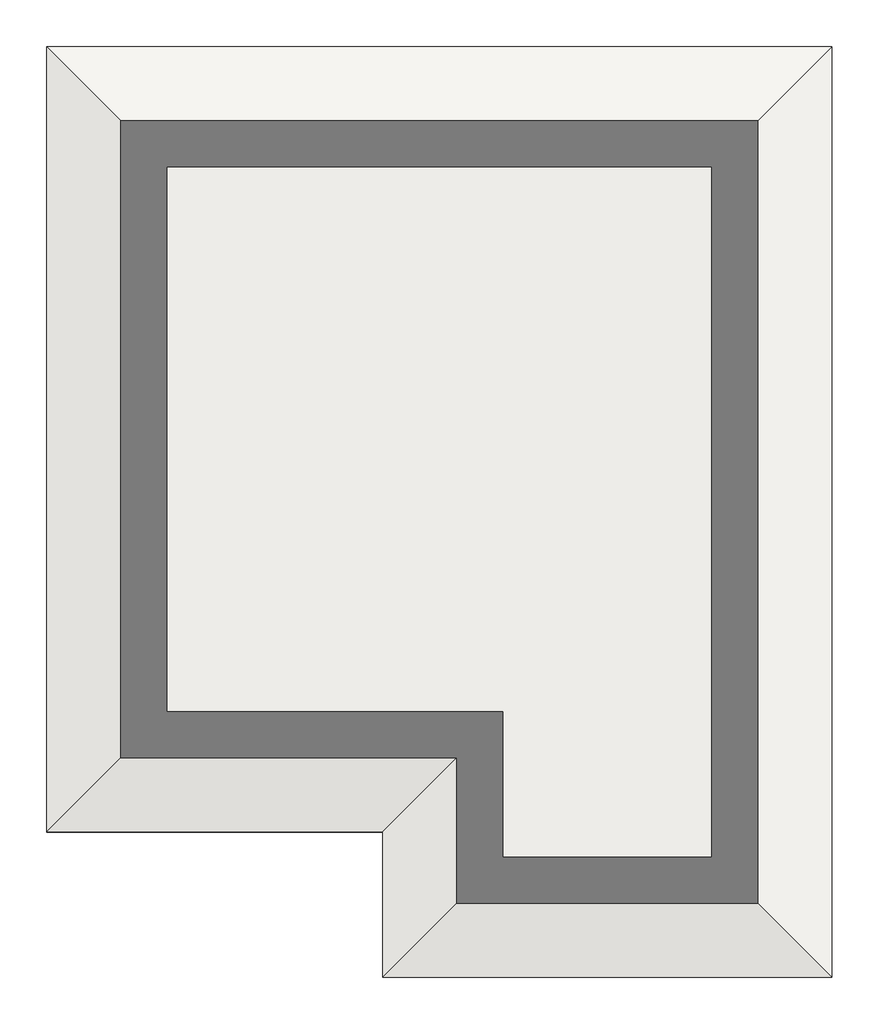
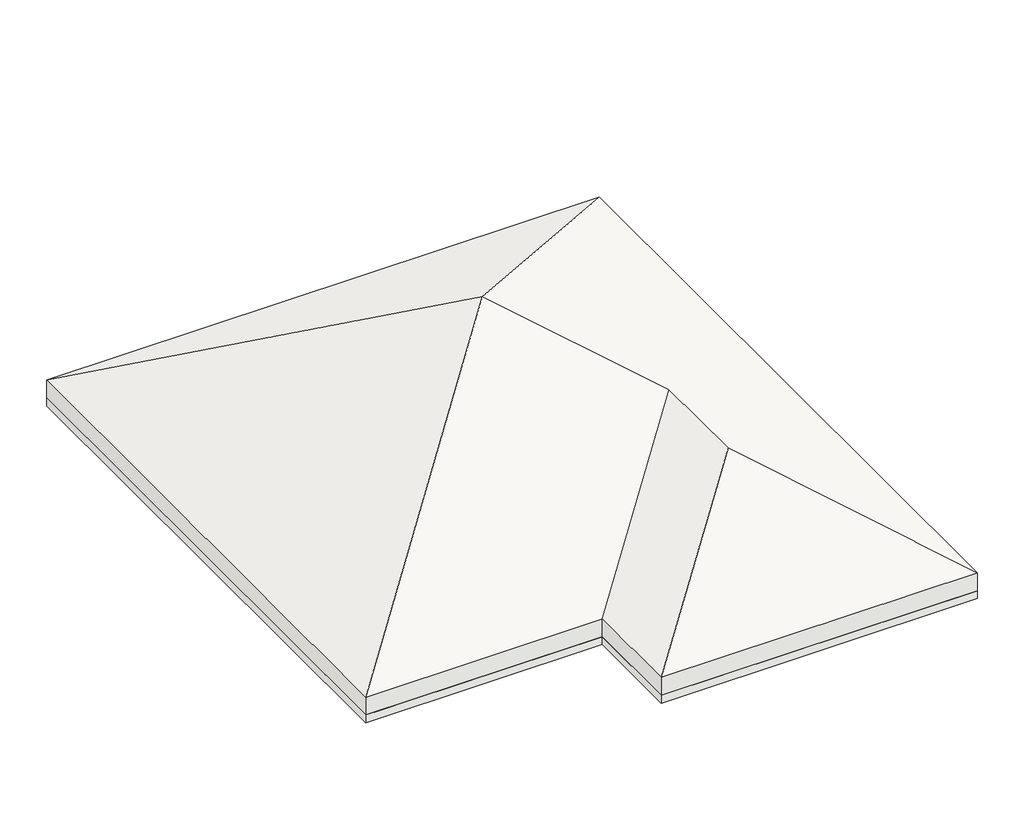
# One storey: 15 beams, 6 walls, 1 roof, 1 slab.
"""IFC4 building model written with IfcOpenShell, lengths in millimetres."""

from ifc_helpers import new_model, si_unit, frame, origin, place, context, project, spatial, polyline, outline, extrude, faceted_brep, element, save

model = new_model("IFC4")

# Units and contexts
model_context = context("Model", 3, world=origin())
ifc_project = project(units=[si_unit("LENGTHUNIT", "METRE", prefix="MILLI")], contexts=[model_context])

# Site, building, storey
site = spatial("IfcSite", under=ifc_project)
building = spatial("IfcBuilding", under=site)
storey = spatial("IfcBuildingStorey", under=building, Name="02 Çatı Katı", Elevation=100780.0)

# Beams
placement = place(None, origin())
element("IfcBeam", 1, ObjectType="M_Concrete-Rectangular Beam : 45x60cm Kiriş", at=placement, inside=storey, context=model_context, shape_type="SweptSolid", body=[
    extrude(outline(polyline([(450.0, 15000.0), (6225.0, 15000.0), (6225.0, 14999.2150597), (5700.0, 14999.2150597), (5700.0, 14550.0), (450.0, 14550.0), (450.0, 15000.0)])), frame((0.0, 0.0, 100180.0), z_axis=(0.0, 0.0, 1.0), x_axis=(1.0, 0.0, 0.0)), (0.0, 0.0, 1.0), 400.0),
])
element("IfcBeam", 2, ObjectType="M_Concrete-Rectangular Beam : 45x60cm Kiriş", at=placement, inside=storey, context=model_context, shape_type="SweptSolid", body=[
    extrude(outline(polyline([(450.0, 8750.0), (5775.0, 8750.0), (5775.0, 8300.0), (450.0, 8300.0), (450.0, 8750.0)])), frame((0.0, 0.0, 100180.0), z_axis=(0.0, 0.0, 1.0), x_axis=(1.0, 0.0, 0.0)), (0.0, 0.0, 1.0), 400.0),
])
element("IfcBeam", 3, ObjectType="M_Concrete-Rectangular Beam : 45x60cm Kiriş", at=placement, inside=storey, context=model_context, shape_type="SweptSolid", body=[
    extrude(outline(polyline([(0.0, 8800.0), (0.0, 14400.0), (450.0, 14400.0), (450.0, 8800.0), (0.0, 8800.0)])), frame((0.0, 0.0, 100180.0), z_axis=(0.0, 0.0, 1.0), x_axis=(1.0, 0.0, 0.0)), (0.0, 0.0, 1.0), 400.0),
])
element("IfcBeam", 4, ObjectType="M_Concrete-Rectangular Beam : 45x60cm Kiriş", at=placement, inside=storey, context=model_context, shape_type="SweptSolid", body=[
    extrude(outline(polyline([(0.0, 3100.0), (0.0, 8200.0), (450.0, 8200.0), (450.0, 3100.0), (0.0, 3100.0)])), frame((0.0, 0.0, 100180.0), z_axis=(0.0, 0.0, 1.0), x_axis=(1.0, 0.0, 0.0)), (0.0, 0.0, 1.0), 400.0),
])
element("IfcBeam", 5, ObjectType="M_Concrete-Rectangular Beam : 45x60cm Kiriş", at=placement, inside=storey, context=model_context, shape_type="SweptSolid", body=[
    extrude(outline(polyline([(5700.0, 2500.0), (450.0, 2500.0), (450.0, 2950.0), (5700.0, 2950.0), (5700.0, 2500.0)])), frame((0.0, 0.0, 100180.0), z_axis=(0.0, 0.0, 1.0), x_axis=(1.0, 0.0, 0.0)), (0.0, 0.0, 1.0), 400.0),
])
element("IfcBeam", 6, ObjectType="M_Concrete-Rectangular Beam : 45x60cm Kiriş", at=placement, inside=storey, context=model_context, shape_type="SweptSolid", body=[
    extrude(outline(polyline([(12050.0, 2500.0), (6300.0, 2500.0), (6300.0, 2950.0), (12050.0, 2950.0), (12050.0, 2500.0)])), frame((0.0, 0.0, 100180.0), z_axis=(0.0, 0.0, 1.0), x_axis=(1.0, 0.0, 0.0)), (0.0, 0.0, 1.0), 400.0),
])
element("IfcBeam", 7, ObjectType="M_Concrete-Rectangular Beam : 45x60cm Kiriş", at=placement, inside=storey, context=model_context, shape_type="SweptSolid", body=[
    extrude(outline(polyline([(12500.0, 8750.0), (12500.0, 3100.0), (12050.0, 3100.0), (12050.0, 8200.0), (12494.8117928, 8200.0), (12494.8117928, 8750.0), (12500.0, 8750.0)])), frame((0.0, 0.0, 100180.0), z_axis=(0.0, 0.0, 1.0), x_axis=(1.0, 0.0, 0.0)), (0.0, 0.0, 1.0), 400.0),
])
element("IfcBeam", 8, ObjectType="M_Concrete-Rectangular Beam : 45x60cm Kiriş", at=placement, inside=storey, context=model_context, shape_type="SweptSolid", body=[
    extrude(outline(polyline([(12032.1117928, 8750.0), (12032.1117928, 8300.0), (6237.7, 8300.0), (6237.7, 8750.0), (12032.1117928, 8750.0)])), frame((0.0, 0.0, 100180.0), z_axis=(0.0, 0.0, 1.0), x_axis=(1.0, 0.0, 0.0)), (0.0, 0.0, 1.0), 400.0),
])
element("IfcBeam", 9, ObjectType="M_Concrete-Rectangular Beam : 30x60cm Kiriş", at=placement, inside=storey, context=model_context, shape_type="SweptSolid", body=[
    extrude(outline(polyline([(9850.0, 15000.0), (9850.0, 14700.0), (6300.0, 14700.0), (6300.0, 15000.0), (9850.0, 15000.0)])), frame((0.0, 0.0, 100180.0), z_axis=(0.0, 0.0, 1.0), x_axis=(1.0, 0.0, 0.0)), (0.0, 0.0, 1.0), 400.0),
])
element("IfcBeam", 10, ObjectType="M_Concrete-Rectangular Beam : 30x60cm Kiriş", at=placement, inside=storey, context=model_context, shape_type="SweptSolid", body=[
    extrude(outline(polyline([(12200.0, 10850.0), (12500.0, 10850.0), (12500.0, 8800.0), (12200.0, 8800.0), (12200.0, 10850.0)])), frame((0.0, 0.0, 100180.0), z_axis=(0.0, 0.0, 1.0), x_axis=(1.0, 0.0, 0.0)), (0.0, 0.0, 1.0), 400.0),
])
element("IfcBeam", 11, ObjectType="M_Concrete-Rectangular Beam : 45x60cm Kiriş", at=placement, inside=storey, context=model_context, shape_type="SweptSolid", body=[
    extrude(outline(polyline([(5775.0, 2950.0), (5775.0, 8200.0), (6225.0, 8200.0), (6225.0, 2950.0), (5775.0, 2950.0)])), frame((0.0, 0.0, 100180.0), z_axis=(0.0, 0.0, 1.0), x_axis=(1.0, 0.0, 0.0)), (0.0, 0.0, 1.0), 400.0),
])
element("IfcBeam", 12, ObjectType="M_Concrete-Rectangular Beam : 45x60cm Kiriş", at=placement, inside=storey, context=model_context, shape_type="SweptSolid", body=[
    extrude(outline(polyline([(5775.0, 14536.5150597), (6225.0, 14536.5150597), (6225.0, 8800.0), (5775.0, 8800.0), (5775.0, 14536.5150597)])), frame((0.0, 0.0, 100180.0), z_axis=(0.0, 0.0, 1.0), x_axis=(1.0, 0.0, 0.0)), (0.0, 0.0, 1.0), 400.0),
])
element("IfcBeam", 13, ObjectType="M_Concrete-Rectangular Beam : 45x60cm Kiriş", at=placement, inside=storey, context=model_context, shape_type="Brep", body=[
    faceted_brep([(5775.0, 2500.0, 100180.0), (5775.0, 400.0, 100180.0), (5775.0, 400.0, 100580.0), (5775.0, 2500.0, 100580.0), (6225.0, 2500.0, 100180.0), (6225.0, 450.0, 100180.0), (6225.0, 0.0, 100180.0), (6175.0, 0.0, 100180.0), (6175.0, 400.0, 100180.0), (6225.0, 2500.0, 100580.0), (6225.0, 450.0, 100580.0), (6225.0, 0.0, 100580.0), (6175.0, 0.0, 100580.0), (6175.0, 400.0, 100580.0)], [[[0, 1, 2, 3]], [[0, 4, 5, 6, 7, 8, 1]], [[6, 5, 4, 9, 10, 11]], [[4, 0, 3, 9]], [[8, 7, 12, 13]], [[1, 8, 13, 2]], [[3, 2, 13, 12, 11, 10, 9]], [[7, 6, 11, 12]]]),
])
element("IfcBeam", 14, ObjectType="M_Concrete-Rectangular Beam : 45x60cm Kiriş", at=placement, inside=storey, context=model_context, shape_type="Brep", body=[
    faceted_brep([(6225.0, 0.0, 100580.0), (6225.0, 0.0, 100180.0), (12100.0, 0.0, 100180.0), (12100.0, 0.0, 100580.0), (6225.0, 450.0, 100180.0), (12050.0, 450.0, 100180.0), (12500.0, 450.0, 100180.0), (12500.0, 400.0, 100180.0), (12100.0, 400.0, 100180.0), (6225.0, 450.0, 100580.0), (12050.0, 450.0, 100580.0), (12500.0, 450.0, 100580.0), (12100.0, 400.0, 100580.0), (12500.0, 400.0, 100580.0)], [[[0, 1, 2, 3]], [[1, 4, 5, 6, 7, 8, 2]], [[4, 9, 10, 11, 6, 5]], [[4, 1, 0, 9]], [[11, 10, 9, 0, 3, 12, 13]], [[6, 11, 13, 7]], [[8, 12, 3, 2]], [[12, 8, 7, 13]]]),
])
element("IfcBeam", 15, ObjectType="M_Concrete-Rectangular Beam : 45x60cm Kiriş", at=placement, inside=storey, context=model_context, shape_type="SweptSolid", body=[
    extrude(outline(polyline([(12050.0, 2500.0), (12500.0, 2500.0), (12500.0, 450.0), (12050.0, 450.0), (12050.0, 2500.0)])), frame((0.0, 0.0, 100180.0), z_axis=(0.0, 0.0, 1.0), x_axis=(1.0, 0.0, 0.0)), (0.0, 0.0, 1.0), 400.0),
])

# Roof
element("IfcRoof", 16, ObjectType="Generic - 400mm", at=placement, inside=storey, context=model_context, shape_type="Brep", body=[
    faceted_brep([(5275.0, -500.0, 100780.0), (9137.5, 3362.5, 103010.0154147), (13000.0, -500.0, 100780.0), (5275.0, 2000.0, 100780.0), (9137.5, 5862.5, 103010.0154147), (-500.0, 2000.0, 100780.0), (6250.0, 8750.0, 104677.114317), (-500.0, 15500.0, 100780.0), (13000.0, 15500.0, 100780.0), (5275.0, -500.0, 101241.8802154), (13000.0, -500.0, 101241.8802154), (9137.5, 3362.5, 103471.8956301), (5275.0, 2000.0, 101241.8802154), (9137.5, 5862.5, 103471.8956301), (-500.0, 2000.0, 101241.8802154), (6250.0, 8750.0, 105138.9945324), (-500.0, 15500.0, 101241.8802154), (13000.0, 15500.0, 101241.8802154)], [[[0, 1, 2]], [[0, 3, 4, 1]], [[5, 6, 4, 3]], [[7, 6, 5]], [[6, 7, 8]], [[2, 1, 4, 6, 8]], [[9, 10, 11]], [[12, 9, 11, 13]], [[14, 12, 13, 15]], [[16, 14, 15]], [[16, 15, 17]], [[10, 17, 15, 13, 11]], [[5, 14, 16, 7]], [[3, 12, 14, 5]], [[0, 9, 12, 3]], [[2, 10, 9, 0]], [[8, 17, 10, 2]], [[7, 16, 17, 8]]]),
])

# Slab
element("IfcSlab", 17, ObjectType="20cm Döşeme", at=placement, inside=storey, context=model_context, shape_type="SweptSolid", body=[
    extrude(outline(polyline([(13000.0, 15500.0), (13000.0, -500.0), (5275.0, -500.0), (5275.0, 2000.0), (-500.0, 2000.0), (-500.0, 15500.0), (13000.0, 15500.0)])), frame((0.0, 0.0, 100580.0), z_axis=(0.0, 0.0, 1.0), x_axis=(1.0, 0.0, 0.0)), (0.0, 0.0, 1.0), 200.0),
])

# Walls
element("IfcWall", 18, ObjectType="25cm Perde Duvar", at=placement, inside=storey, context=model_context, shape_type="Brep", body=[
    faceted_brep([(-250.0, 15500.0, 100780.0), (-250.0, 15250.0, 100924.3375673), (-250.0, 2250.0, 100924.3375673), (-250.0, 2000.0, 100780.0), (-250.0, 2250.0, 100780.0), (-250.0, 15250.0, 100780.0), (-500.0, 2000.0, 100780.0), (-500.0, 15500.0, 100780.0)], [[[0, 1, 2, 3, 4, 5]], [[6, 7, 0, 5, 4, 3]], [[7, 6, 2, 1]], [[6, 3, 2]], [[1, 0, 7]]]),
])
element("IfcWall", 19, ObjectType="25cm Perde Duvar", at=placement, inside=storey, context=model_context, shape_type="SweptSolid", body=[
    extrude(outline(polyline([(2250.0, 100780.0), (2000.0, 100780.0), (2250.0, 100924.3375673), (2250.0, 100780.0)])), frame((-250.0, 0.0, 0.0), z_axis=(1.0, 0.0, 0.0), x_axis=(0.0, 1.0, 0.0)), (0.0, 0.0, 1.0), 5775.0),
])
element("IfcWall", 20, ObjectType="25cm Perde Duvar", at=placement, inside=storey, context=model_context, shape_type="Brep", body=[
    faceted_brep([(5525.0, 2000.0, 100780.0), (5525.0, 2000.0, 100924.3375673), (5525.0, -250.0, 100924.3375673), (5525.0, -500.0, 100780.0), (5525.0, -250.0, 100780.0), (5275.0, -500.0, 100780.0), (5275.0, 2000.0, 100780.0)], [[[0, 1, 2, 3, 4]], [[5, 6, 0, 4, 3]], [[6, 1, 0]], [[6, 5, 2, 1]], [[5, 3, 2]]]),
])
element("IfcWall", 21, ObjectType="25cm Perde Duvar", at=placement, inside=storey, context=model_context, shape_type="Brep", body=[
    faceted_brep([(5525.0, -250.0, 100780.0), (5525.0, -250.0, 100924.3375673), (12750.0, -250.0, 100924.3375673), (13000.0, -250.0, 100780.0), (12750.0, -250.0, 100780.0), (13000.0, -500.0, 100780.0), (5525.0, -500.0, 100780.0)], [[[0, 1, 2, 3, 4]], [[5, 6, 0, 4, 3]], [[6, 1, 0]], [[6, 5, 2, 1]], [[5, 3, 2]]]),
])
element("IfcWall", 22, ObjectType="25cm Perde Duvar", at=placement, inside=storey, context=model_context, shape_type="Brep", body=[
    faceted_brep([(12750.0, -250.0, 100780.0), (12750.0, -250.0, 100924.3375673), (12750.0, 15250.0, 100924.3375673), (12750.0, 15500.0, 100780.0), (12750.0, 15250.0, 100780.0), (13000.0, 15500.0, 100780.0), (13000.0, -250.0, 100780.0)], [[[0, 1, 2, 3, 4]], [[5, 6, 0, 4, 3]], [[6, 1, 0]], [[6, 5, 2, 1]], [[5, 3, 2]]]),
])
element("IfcWall", 23, ObjectType="25cm Perde Duvar", at=placement, inside=storey, context=model_context, shape_type="SweptSolid", body=[
    extrude(outline(polyline([(15500.0, 100780.0), (15250.0, 100780.0), (15250.0, 100924.3375673), (15500.0, 100780.0)])), frame((-250.0, 0.0, 0.0), z_axis=(1.0, 0.0, 0.0), x_axis=(0.0, 1.0, 0.0)), (0.0, 0.0, 1.0), 13000.0),
])

save(model, "model.ifc")

# Revit data of these elements
# Type "M_Concrete-Rectangular Beam : 45x60cm Kiriş"
#   Length [instance default] = 152.40 cm
#   b = 45.00 cm
#   h = 60.00 cm
#   Structural Material [instance default] = Concrete, Cast-in-Place gray
#   Assembly Code = ""
# Type "M_Concrete-Rectangular Beam : 30x60cm Kiriş"
#   Length [instance default] = 152.40 cm
#   b = 30.00 cm
#   h = 60.00 cm
#   Structural Material [instance default] = Concrete, Cast-in-Place gray
#   Assembly Code = ""
# Type "Generic - 400mm"
#   Layers, outside or top first: 40.00 cm no material (function 1)
# Type "20cm Döşeme"
#   Function = 0
#   Layers, outside or top first: 20.00 cm "Concrete, Cast In Situ" (function 1)
# Type "25cm Perde Duvar"
#   Layers, outside or top first: 25.00 cm "Concrete, Cast In Situ" (function 1)
# Elements 1, 2, 3, 4, 5, 6, 7, 8, 11, 12, 13, 14, 15 (IfcBeam, "M_Concrete-Rectangular Beam : 45x60cm Kiriş")
#   Comments = ""
#   Structural Material = Concrete, Cast-in-Place gray
#   Phase Created = New Construction
#   Materials on its faces: "Concrete, Cast-in-Place gray"
# Elements 9, 10 (IfcBeam, "M_Concrete-Rectangular Beam : 30x60cm Kiriş")
#   Comments = ""
#   Structural Material = Concrete, Cast-in-Place gray
#   Phase Created = New Construction
#   Materials on its faces: "Concrete, Cast-in-Place gray"
# Element 16 (IfcRoof, "Generic - 400mm")
#   built-in parameter 1001705 = 344.944 (stored number, unit not read)
#   built-in parameter 1001710 = 33615
#   Phase Created = New Construction
#   Materials on its faces: "Default Roof"
# Element 17 (IfcSlab, "20cm Döşeme")
#   Height Offset From Level = 0.00 cm
#   built-in parameter 1001954 = 1
#   Phase Created = New Construction
#   Materials on its faces: "Concrete, Cast In Situ"
# Elements 18, 19, 20, 21, 22, 23 (IfcWall, "25cm Perde Duvar")
#   Comments = ""
#   Top Offset = 0.00 cm
#   Base Offset = 0.00 cm
#   Unconnected Height = 60.00 cm
#   wall height = 60.00 cm
#   Phase Created = New Construction
#   Base Constraint = 02 Çatı Katı
#   Materials on its faces: "Concrete, Cast In Situ"
# Materials
#   "Concrete, Cast-in-Place gray": class "Concrete", colour RGB 192 192 192, transparency 0, Description = "Cast-in-place concrete", Cost = 0
#   "Concrete, Cast In Situ": class "Concrete", colour RGB 192 192 192, transparency 0, Description = "physical material", Cost = 0
#   "Default Roof": class "Miscellaneous", colour RGB 0 127 0, transparency 0
